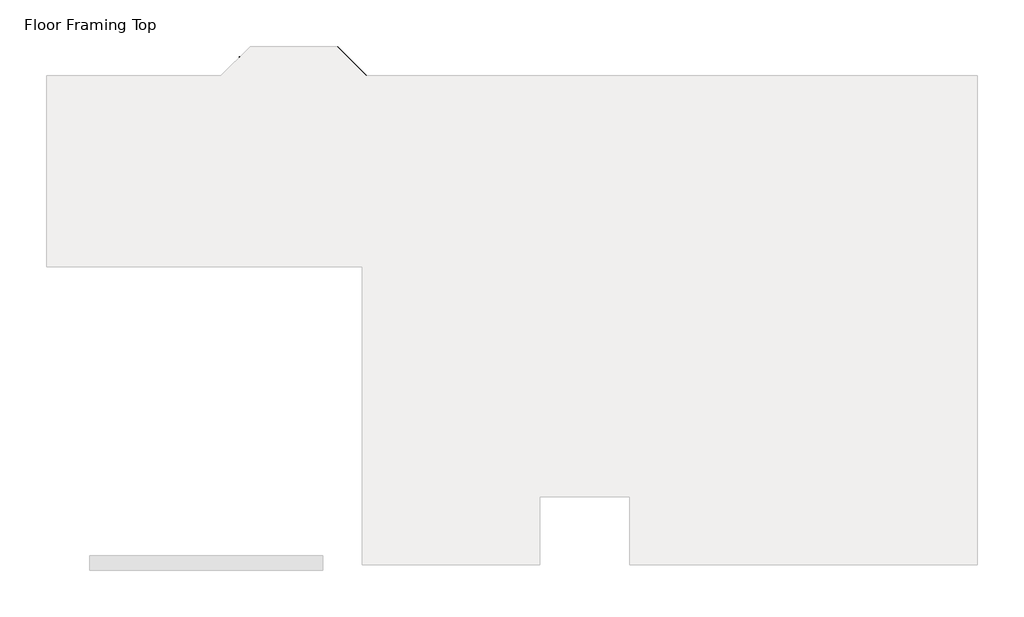
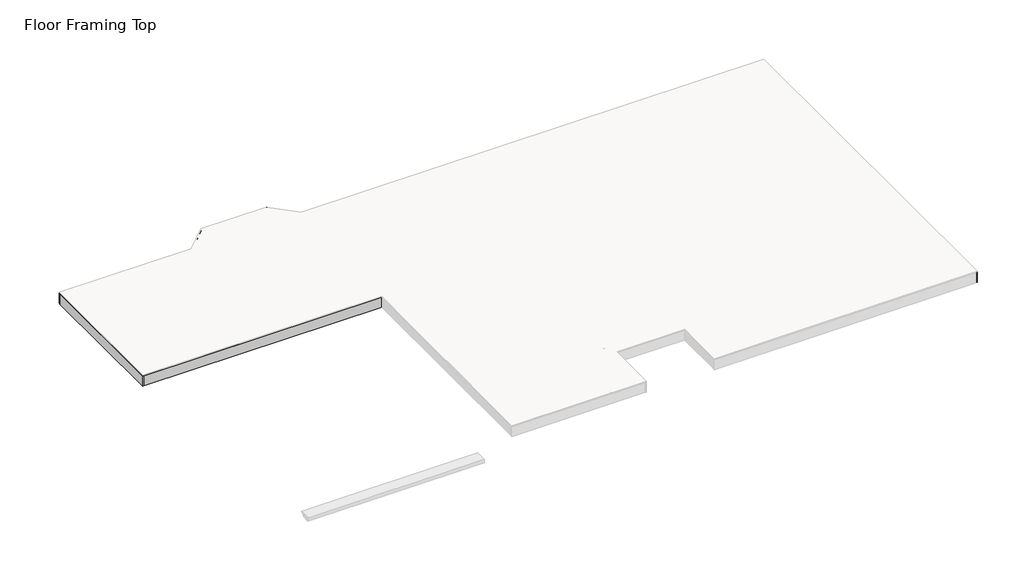
# One storey, part 4 of 4: 30 beams.
"""IFC4 building model written with IfcOpenShell, lengths in millimetres."""

import ifcopenshell
import ifcopenshell.guid

model = None  # the IFC model being written
_history = None  # IfcOwnerHistory: only IFC2X3 demands one
_inside = {}  # id of a spatial element -> (the spatial element, [elements in it])
_under = {}  # id of a project, library or spatial element -> (it, [spatial elements below it])
_declared = {}  # id of a project -> (the project, [libraries it declares])
_typed = {}  # id of a type object -> (the type object, [elements of that type])
_made_of = {}  # id of a material, layer set ... -> (it, [elements and type objects made of it])


def new_model(schema):
    """Start an empty IFC model of exactly this schema.

    Asked for "IFC4X3", IfcOpenShell would pick the latest addendum, in which some entities
    have other attributes; the version numbers below select the first issue.
    IFC2X3 requires an IfcOwnerHistory on every rooted entity: one is made here for all.
    """
    global model, _history
    if schema == "IFC4X3":
        model = ifcopenshell.file(schema_version=(4, 3, 0, 0))
    else:
        model = ifcopenshell.file(schema=schema)
    _inside.clear()
    _under.clear()
    _declared.clear()
    _typed.clear()
    _made_of.clear()
    _history = None
    if model.schema == "IFC2X3":
        org = make("IfcOrganization", Name="unknown")
        user = make(
            "IfcPersonAndOrganization",
            ThePerson=make("IfcPerson", FamilyName="unknown"),
            TheOrganization=org,
        )
        app = make(
            "IfcApplication",
            ApplicationDeveloper=org,
            Version="unknown",
            ApplicationFullName="unknown",
            ApplicationIdentifier="unknown",
        )
        _history = make(
            "IfcOwnerHistory",
            OwningUser=user,
            OwningApplication=app,
            ChangeAction="ADDED",
            CreationDate=0,
        )
    return model


def make(cls, **values):
    """One entity of the class cls with the attributes given. An attribute that is None is left unset."""
    return model.create_entity(
        cls, **{name: value for name, value in values.items() if value is not None}
    )


def rooted(cls, **values):
    """An entity with a GlobalId (a new one), such as an element, a storey or a relation."""
    return make(cls, GlobalId=ifcopenshell.guid.new(), OwnerHistory=_history, **values)


def si_unit(unit_type, name, prefix=None):
    """IfcSIUnit, for example si_unit("LENGTHUNIT", "METRE", prefix="MILLI")."""
    return make("IfcSIUnit", UnitType=unit_type, Prefix=prefix, Name=name)


def assignment(units):
    """IfcUnitAssignment: the units of a project."""
    return None if units is None else make("IfcUnitAssignment", Units=units)


def point(xyz):
    """IfcCartesianPoint."""
    return None if xyz is None else make("IfcCartesianPoint", Coordinates=xyz)


def direction(xyz):
    """IfcDirection."""
    return None if xyz is None else make("IfcDirection", DirectionRatios=xyz)


def frame(location, z_axis=None, x_axis=None):
    """IfcAxis2Placement3D, a coordinate frame: its origin and axes. An axis left out is left unset."""
    return make(
        "IfcAxis2Placement3D",
        Location=point(location),
        Axis=direction(z_axis),
        RefDirection=direction(x_axis),
    )


def origin():
    """The frame at (0, 0, 0) with its axes left unset."""
    return frame((0.0, 0.0, 0.0))


def place(relative_to, where):
    """IfcLocalPlacement: puts the frame where relative to a parent placement (None: the world)."""
    return make(
        "IfcLocalPlacement", PlacementRelTo=relative_to, RelativePlacement=where
    )


def context(
    kind, dimensions, precision=None, world=None, true_north=None, identifier=None
):
    """IfcGeometricRepresentationContext, for example the 3D "Model" context."""
    return make(
        "IfcGeometricRepresentationContext",
        ContextIdentifier=identifier,
        ContextType=kind,
        CoordinateSpaceDimension=dimensions,
        Precision=precision,
        WorldCoordinateSystem=world,
        TrueNorth=true_north,
    )


def project(units=None, contexts=None):
    """IfcProject with its units and contexts."""
    return rooted(
        "IfcProject",
        Name="project",
        RepresentationContexts=contexts,
        UnitsInContext=assignment(units),
    )


def spatial(cls, under=None, at=None, **own):
    """A site, building, storey or space (cls), placed at a placement, below another one or the project."""
    s = rooted(cls, ObjectPlacement=at, **own)
    if under is not None:
        _under.setdefault(under.id(), (under, []))[1].append(s)
    return s


def polyline(points):
    """IfcPolyline through the points."""
    return make("IfcPolyline", Points=[point(p) for p in points])


def outline(outer, holes=None, kind="AREA"):
    """IfcArbitraryClosedProfileDef: a profile drawn as a closed curve; with holes, ...WithVoids."""
    if holes is None:
        return make("IfcArbitraryClosedProfileDef", ProfileType=kind, OuterCurve=outer)
    return make(
        "IfcArbitraryProfileDefWithVoids",
        ProfileType=kind,
        OuterCurve=outer,
        InnerCurves=holes,
    )


def extrude(swept, where, along, depth):
    """IfcExtrudedAreaSolid: the profile swept, set in the frame where, extruded along a direction by depth."""
    return make(
        "IfcExtrudedAreaSolid",
        SweptArea=swept,
        Position=where,
        ExtrudedDirection=direction(along),
        Depth=depth,
    )


def faces_of(points, faces, orient=None, outer=None):
    """IfcFace entities. A face is a list of loops; a loop is a list of indices into points, from 0.

    orient and outer hold one flag for each loop. By default every Orientation is true, the
    first loop of a face is its IfcFaceOuterBound and the others are IfcFaceBound.
    """
    made = []
    for i, loops in enumerate(faces):
        bounds = []
        for j, loop in enumerate(loops):
            is_outer = j == 0 if outer is None else outer[i][j]
            bounds.append(
                make(
                    "IfcFaceOuterBound" if is_outer else "IfcFaceBound",
                    Bound=make("IfcPolyLoop", Polygon=[points[k] for k in loop]),
                    Orientation=True if orient is None else orient[i][j],
                )
            )
        made.append(make("IfcFace", Bounds=bounds))
    return made


def faceted_brep(points, faces, orient=None, outer=None, voids=None):
    """IfcFacetedBrep: a solid bounded by flat faces; with voids (closed shells), ...WithVoids."""
    shared = [point(p) for p in points]
    hull = make("IfcClosedShell", CfsFaces=faces_of(shared, faces, orient, outer))
    if voids is None:
        return make("IfcFacetedBrep", Outer=hull)
    return make(
        "IfcFacetedBrepWithVoids",
        Outer=hull,
        Voids=[
            make(cls, CfsFaces=faces_of(shared, fs, o, b)) for cls, fs, o, b in voids
        ],
    )


def shape(context_of_items, identifier, shape_type, items):
    """IfcShapeRepresentation: the items that make up one representation, for example the "Body"."""
    return make(
        "IfcShapeRepresentation",
        ContextOfItems=context_of_items,
        RepresentationIdentifier=identifier,
        RepresentationType=shape_type,
        Items=items,
    )


def source(mapping_origin, context_of_items, identifier, shape_type, items):
    """IfcRepresentationMap: a shape defined once, which mapped items show again and again."""
    return make(
        "IfcRepresentationMap",
        MappingOrigin=mapping_origin,
        MappedRepresentation=shape(context_of_items, identifier, shape_type, items),
    )


def transform(
    local_origin,
    x_axis=None,
    y_axis=None,
    z_axis=None,
    scale=None,
    scale2=None,
    scale3=None,
    uniform=True,
):
    """IfcCartesianTransformationOperator3D, or its non-uniform kind. x_axis, y_axis, z_axis: its Axis1, 2, 3."""
    if uniform:
        return make(
            "IfcCartesianTransformationOperator3D",
            Axis1=direction(x_axis),
            Axis2=direction(y_axis),
            LocalOrigin=point(local_origin),
            Scale=scale,
            Axis3=direction(z_axis),
        )
    return make(
        "IfcCartesianTransformationOperator3DnonUniform",
        Axis1=direction(x_axis),
        Axis2=direction(y_axis),
        LocalOrigin=point(local_origin),
        Scale=scale,
        Axis3=direction(z_axis),
        Scale2=scale2,
        Scale3=scale3,
    )


def mapped(mapping_source, mapping_target):
    """IfcMappedItem: shows the shape of a source again, moved by a transform."""
    return make(
        "IfcMappedItem", MappingSource=mapping_source, MappingTarget=mapping_target
    )


def made_of(thing, what):
    """Note that an element or type object is made of a material, layer set ...; save() writes the relation."""
    if what is not None:
        _made_of.setdefault(what.id(), (what, []))[1].append(thing)
    return thing


def element(
    cls,
    number,
    at=None,
    inside=None,
    cuts=None,
    type_object=None,
    material=None,
    context=None,
    identifier="Body",
    shape_type=None,
    held_by="IfcProductDefinitionShape",
    body=None,
    shapes=None,
    **own,
):
    """One element of the class cls, such as IfcWall. Its Tag is "e" and its number.

    at: its placement. inside: the storey or other place that contains it. cuts: it is an
    opening in that element (IfcRelVoidsElement). A single representation is given by context,
    identifier, shape_type and body (its items); several are given by shapes. held_by: the class
    of the entity that holds the representations. save() writes the other relations.
    """
    e = rooted(cls, Tag="e%d" % number, ObjectPlacement=at, **own)
    if body is not None:
        shapes = [shape(context, identifier, shape_type, body)]
    if shapes is not None:
        e.Representation = make(held_by, Representations=shapes)
    if inside is not None:
        _inside.setdefault(inside.id(), (inside, []))[1].append(e)
    if cuts is not None:
        rooted(
            "IfcRelVoidsElement", RelatingBuildingElement=cuts, RelatedOpeningElement=e
        )
    if type_object is not None:
        _typed.setdefault(type_object.id(), (type_object, []))[1].append(e)
    return made_of(e, material)


def aggregate(whole, parts):
    """IfcRelAggregates: a whole, such as a stair, and the parts it consists of."""
    return rooted("IfcRelAggregates", RelatingObject=whole, RelatedObjects=parts)


def save(model, path):
    """Write the relations noted so far, then the file.

    IfcRelAggregates (storeys below a building ...), IfcRelContainedInSpatialStructure (elements
    in a storey), IfcRelDefinesByType, IfcRelAssociatesMaterial and IfcRelDeclares: one each for
    every whole, place, type object, material and project.
    """
    for whole, parts in _under.values():
        aggregate(whole, parts)
    for where, things in _inside.values():
        rooted(
            "IfcRelContainedInSpatialStructure",
            RelatedElements=things,
            RelatingStructure=where,
        )
    for kind, things in _typed.values():
        rooted("IfcRelDefinesByType", RelatedObjects=things, RelatingType=kind)
    for what, things in _made_of.values():
        rooted("IfcRelAssociatesMaterial", RelatedObjects=things, RelatingMaterial=what)
    for by, libraries in _declared.values():
        rooted("IfcRelDeclares", RelatingContext=by, RelatedDefinitions=libraries)
    model.write(path)


def lvl_laminated_veneer_lumber_rim_board_13dc89ba(model_context):
    return source(origin(), model_context, "Body", "SweptSolid", [
        extrude(outline(polyline([(1981.99375, 15.875), (1981.99375, -15.875), (-1985.16875, -15.875), (-1985.16875, 15.875), (1981.99375, 15.875)])), frame((0.0, 0.0, -150.8125), z_axis=(0.0, 0.0, 1.0), x_axis=(1.0, 0.0, 0.0)), (0.0, 0.0, 1.0), 301.625),
    ])


def lvl_laminated_veneer_lumber_rim_board_6caa49f5(model_context):
    return source(origin(), model_context, "Body", "SweptSolid", [
        extrude(outline(polyline([(3288.50625, 15.875), (3288.50625, -15.875), (-3288.50625, -15.875), (-3288.50625, 15.875), (3288.50625, 15.875)])), frame((0.0, 0.0, -150.8125), z_axis=(0.0, 0.0, 1.0), x_axis=(1.0, 0.0, 0.0)), (0.0, 0.0, 1.0), 301.625),
    ])


def lvl_laminated_veneer_lumber_rim_board_c76fbf88(model_context):
    return source(origin(), model_context, "Body", "SweptSolid", [
        extrude(outline(polyline([(5118.89375, 15.875), (5118.89375, -15.875), (-5118.89375, -15.875), (-5118.89375, 15.875), (5118.89375, 15.875)])), frame((0.0, 0.0, -150.8125), z_axis=(0.0, 0.0, 1.0), x_axis=(1.0, 0.0, 0.0)), (0.0, 0.0, 1.0), 301.625),
    ])


def plywood_web_joist_11_7_8_tji_150_914fbb7f(model_context):
    return source(origin(), model_context, "Body", "SweptSolid", [
        extrude(outline(polyline([(-19.05, 150.8125), (19.05, 150.8125), (19.05, 112.7125), (4.7625, 112.7125), (4.7625, 119.0625), (-4.7625, 119.0625), (-4.7625, 112.7125), (-19.05, 112.7125), (-19.05, 150.8125)])), frame((-2272.50625, 0.0, 0.0), z_axis=(1.0, 0.0, 0.0), x_axis=(0.0, 1.0, 0.0)), (0.0, 0.0, 1.0), 4545.0125),
        extrude(outline(polyline([(19.05, -112.7125), (19.05, -150.8125), (-19.05, -150.8125), (-19.05, -112.7125), (-4.7625, -112.7125), (-4.7625, -118.3285374), (4.7625, -118.3285374), (4.7625, -112.7125), (19.05, -112.7125)])), frame((-2272.50625, 0.0, 0.0), z_axis=(1.0, 0.0, 0.0), x_axis=(0.0, 1.0, 0.0)), (0.0, 0.0, 1.0), 4545.0125),
        extrude(outline(polyline([(2272.50625, 4.7625), (2272.50625, -4.7625), (-2272.50625, -4.7625), (-2272.50625, 4.7625), (2272.50625, 4.7625)])), frame((0.0, 0.0, -118.3285374), z_axis=(0.0, 0.0, 1.0), x_axis=(1.0, 0.0, 0.0)), (0.0, 0.0, 1.0), 237.3910374),
    ])


def plywood_web_joist_11_7_8_tji_150_4ba6f87f(model_context):
    return source(origin(), model_context, "Body", "SweptSolid", [
        extrude(outline(polyline([(-19.05, 150.8125), (19.05, 150.8125), (19.05, 112.7125), (4.7625, 112.7125), (4.7625, 119.0625), (-4.7625, 119.0625), (-4.7625, 112.7125), (-19.05, 112.7125), (-19.05, 150.8125)])), frame((-1967.70625, 0.0, 0.0), z_axis=(1.0, 0.0, 0.0), x_axis=(0.0, 1.0, 0.0)), (0.0, 0.0, 1.0), 3935.4125),
        extrude(outline(polyline([(19.05, -112.7125), (19.05, -150.8125), (-19.05, -150.8125), (-19.05, -112.7125), (-4.7625, -112.7125), (-4.7625, -118.3285374), (4.7625, -118.3285374), (4.7625, -112.7125), (19.05, -112.7125)])), frame((-1967.70625, 0.0, 0.0), z_axis=(1.0, 0.0, 0.0), x_axis=(0.0, 1.0, 0.0)), (0.0, 0.0, 1.0), 3935.4125),
        extrude(outline(polyline([(1967.70625, 4.7625), (1967.70625, -4.7625), (-1967.70625, -4.7625), (-1967.70625, 4.7625), (1967.70625, 4.7625)])), frame((0.0, 0.0, -118.3285374), z_axis=(0.0, 0.0, 1.0), x_axis=(1.0, 0.0, 0.0)), (0.0, 0.0, 1.0), 237.3910374),
    ])


model = new_model("IFC4")

# Units and contexts
model_context = context("Model", 3, world=origin())
ifc_project = project(units=[si_unit("LENGTHUNIT", "METRE", prefix="MILLI")], contexts=[model_context])

# Site, building, storey
site = spatial("IfcSite", under=ifc_project)
building = spatial("IfcBuilding", under=site)
storey = spatial("IfcBuildingStorey", under=building, Name="Floor Framing Top", Elevation=0.0)

# Beams
placement = place(None, origin())
element("IfcBeam", 1, ObjectType="LVL-Laminated Veneer Lumber : Rim Board", at=placement, inside=storey, context=model_context, shape_type="SweptSolid", body=[
    extrude(outline(polyline([(-2583.3027251, 4488.2334053), (-2570.1514445, 4456.4834053), (-6240.9027251, 4456.4834053), (-6240.9027251, 4488.2334053), (-2583.3027251, 4488.2334053)])), frame((0.0, 0.0, -301.625), z_axis=(0.0, 0.0, 1.0), x_axis=(1.0, 0.0, 0.0)), (0.0, 0.0, 1.0), 301.625),
])
element("IfcBeam", 2, ObjectType="LVL-Laminated Veneer Lumber : Rim Board", at=placement, inside=storey, context=model_context, shape_type="SweptSolid", body=[
    extrude(outline(polyline([(-1973.7027251, 5097.8334053), (-1960.5514445, 5066.0834053), (-2570.1514445, 4456.4834053), (-2583.3027251, 4488.2334053), (-1973.7027251, 5097.8334053)])), frame((0.0, 0.0, -301.625), z_axis=(0.0, 0.0, 1.0), x_axis=(1.0, 0.0, 0.0)), (0.0, 0.0, 1.0), 301.625),
])
element("IfcBeam", 3, ObjectType="LVL-Laminated Veneer Lumber : Rim Board", at=placement, inside=storey, context=model_context, shape_type="SweptSolid", body=[
    extrude(outline(polyline([(-144.9027251, 5097.8334053), (-158.0540057, 5066.0834053), (-1960.5514445, 5066.0834053), (-1973.7027251, 5097.8334053), (-144.9027251, 5097.8334053)])), frame((0.0, 0.0, -301.625), z_axis=(0.0, 0.0, 1.0), x_axis=(1.0, 0.0, 0.0)), (0.0, 0.0, 1.0), 301.625),
])
element("IfcBeam", 4, ObjectType="LVL-Laminated Veneer Lumber : Rim Board", at=placement, inside=storey, context=model_context, shape_type="SweptSolid", body=[
    extrude(outline(polyline([(451.5459943, 4456.4834053), (464.6972749, 4488.2334053), (13212.3222749, 4488.2334053), (13212.3222749, 4456.4834053), (451.5459943, 4456.4834053)])), frame((0.0, 0.0, -301.625), z_axis=(0.0, 0.0, 1.0), x_axis=(1.0, 0.0, 0.0)), (0.0, 0.0, 1.0), 301.625),
])
element("IfcBeam", 5, ObjectType="LVL-Laminated Veneer Lumber : Rim Board", at=placement, inside=storey, context=model_context, shape_type="SweptSolid", body=[
    extrude(outline(polyline([(-144.9027251, 5097.8334053), (464.6972749, 4488.2334053), (451.5459943, 4456.4834053), (-158.0540057, 5066.0834053), (-144.9027251, 5097.8334053)])), frame((0.0, 0.0, -301.625), z_axis=(0.0, 0.0, 1.0), x_axis=(1.0, 0.0, 0.0)), (0.0, 0.0, 1.0), 301.625),
])
lvl_laminated_veneer_lumber_rim_board_shape = lvl_laminated_veneer_lumber_rim_board_13dc89ba(model_context)
element("IfcBeam", 6, ObjectType="LVL-Laminated Veneer Lumber : Rim Board", at=placement, inside=storey, context=model_context, shape_type="MappedRepresentation", body=[
    mapped(lvl_laminated_veneer_lumber_rim_board_shape, transform((-6225.0277251, 2471.3146553, -150.8125), x_axis=(0.0, -1.0, 0.0), y_axis=(1.0, 0.0, 0.0), z_axis=(0.0, 0.0, 1.0))),
])
lvl_laminated_veneer_lumber_rim_board_2_shape = lvl_laminated_veneer_lumber_rim_board_6caa49f5(model_context)
element("IfcBeam", 7, ObjectType="LVL-Laminated Veneer Lumber : Rim Board", at=placement, inside=storey, context=model_context, shape_type="MappedRepresentation", body=[
    mapped(lvl_laminated_veneer_lumber_rim_board_2_shape, transform((-2920.6464751, 505.1959053, -150.8125), x_axis=(1.0, 0.0, 0.0), y_axis=(0.0, 1.0, 0.0), z_axis=(0.0, 0.0, 1.0))),
])
lvl_laminated_veneer_lumber_rim_board_3_shape = lvl_laminated_veneer_lumber_rim_board_c76fbf88(model_context)
element("IfcBeam", 8, ObjectType="LVL-Laminated Veneer Lumber : Rim Board", at=placement, inside=storey, context=model_context, shape_type="MappedRepresentation", body=[
    mapped(lvl_laminated_veneer_lumber_rim_board_3_shape, transform((13228.1972749, -630.6603447, -150.8125), x_axis=(0.0, 1.0, 0.0), y_axis=(-1.0, 0.0, 0.0), z_axis=(0.0, 0.0, 1.0))),
])
element("IfcBeam", 9, ObjectType="Plywood Web Joist : 11 7/8 TJI 150", at=placement, inside=storey, context=model_context, shape_type="SweptSolid", body=[
    extrude(outline(polyline([(12040.7472749, -5717.8040947), (12031.2222749, -5717.8040947), (12031.2222749, 4456.4834053), (12040.7472749, 4456.4834053), (12040.7472749, -5717.8040947)])), frame((0.0, 0.0, -269.1410374), z_axis=(0.0, 0.0, 1.0), x_axis=(1.0, 0.0, 0.0)), (0.0, 0.0, 1.0), 237.3910374),
    extrude(outline(polyline([(12031.2222749, -663.2040947), (12031.2222749, 4456.4834053), (12040.7472749, 4456.4834053), (12040.7472749, -663.2040947), (12031.2222749, -663.2040947)])), frame((0.0, 0.0, -269.1410374), z_axis=(0.0, 0.0, 1.0), x_axis=(1.0, 0.0, 0.0)), (0.0, 0.0, 1.0), 237.3910374),
    extrude(outline(polyline([(0.0, 12016.9347749), (-38.1, 12016.9347749), (-38.1, 12031.2222749), (-31.75, 12031.2222749), (-31.75, 12040.7472749), (-38.1, 12040.7472749), (-38.1, 12055.0347749), (0.0, 12055.0347749), (0.0, 12016.9347749)])), frame((0.0, -5717.8040947, 0.0), z_axis=(0.0, 1.0, 0.0), x_axis=(0.0, 0.0, 1.0)), (0.0, 0.0, 1.0), 10174.2875),
    extrude(outline(polyline([(-263.525, 12055.0347749), (-263.525, 12040.7472749), (-269.1410374, 12040.7472749), (-269.1410374, 12031.2222749), (-263.525, 12031.2222749), (-263.525, 12016.9347749), (-301.625, 12016.9347749), (-301.625, 12055.0347749), (-263.525, 12055.0347749)])), frame((0.0, -5717.8040947, 0.0), z_axis=(0.0, 1.0, 0.0), x_axis=(0.0, 0.0, 1.0)), (0.0, 0.0, 1.0), 10174.2875),
    extrude(outline(polyline([(0.0, 12016.9347749), (-38.1, 12016.9347749), (-38.1, 12031.2222749), (-31.75, 12031.2222749), (-31.75, 12040.7472749), (-38.1, 12040.7472749), (-38.1, 12055.0347749), (0.0, 12055.0347749), (0.0, 12016.9347749)])), frame((0.0, -663.2040947, 0.0), z_axis=(0.0, 1.0, 0.0), x_axis=(0.0, 0.0, 1.0)), (0.0, 0.0, 1.0), 5119.6875),
    extrude(outline(polyline([(-263.525, 12055.0347749), (-263.525, 12040.7472749), (-269.1410374, 12040.7472749), (-269.1410374, 12031.2222749), (-263.525, 12031.2222749), (-263.525, 12016.9347749), (-301.625, 12016.9347749), (-301.625, 12055.0347749), (-263.525, 12055.0347749)])), frame((0.0, -663.2040947, 0.0), z_axis=(0.0, 1.0, 0.0), x_axis=(0.0, 0.0, 1.0)), (0.0, 0.0, 1.0), 5119.6875),
])
element("IfcBeam", 10, ObjectType="Plywood Web Joist : 11 7/8 TJI 150", at=placement, inside=storey, context=model_context, shape_type="SweptSolid", body=[
    extrude(outline(polyline([(5944.7472749, -4295.4040947), (5935.2222749, -4295.4040947), (5935.2222749, 4456.4834053), (5944.7472749, 4456.4834053), (5944.7472749, -4295.4040947)])), frame((0.0, 0.0, -269.1410374), z_axis=(0.0, 0.0, 1.0), x_axis=(1.0, 0.0, 0.0)), (0.0, 0.0, 1.0), 237.3910374),
    extrude(outline(polyline([(5935.2222749, -663.2040947), (5935.2222749, 4456.4834053), (5944.7472749, 4456.4834053), (5944.7472749, -663.2040947), (5935.2222749, -663.2040947)])), frame((0.0, 0.0, -269.1410374), z_axis=(0.0, 0.0, 1.0), x_axis=(1.0, 0.0, 0.0)), (0.0, 0.0, 1.0), 237.3910374),
    extrude(outline(polyline([(0.0, 5920.9347749), (-38.1, 5920.9347749), (-38.1, 5935.2222749), (-31.75, 5935.2222749), (-31.75, 5944.7472749), (-38.1, 5944.7472749), (-38.1, 5959.0347749), (0.0, 5959.0347749), (0.0, 5920.9347749)])), frame((0.0, -4295.4040947, 0.0), z_axis=(0.0, 1.0, 0.0), x_axis=(0.0, 0.0, 1.0)), (0.0, 0.0, 1.0), 8751.8875),
    extrude(outline(polyline([(-263.525, 5959.0347749), (-263.525, 5944.7472749), (-269.1410374, 5944.7472749), (-269.1410374, 5935.2222749), (-263.525, 5935.2222749), (-263.525, 5920.9347749), (-301.625, 5920.9347749), (-301.625, 5959.0347749), (-263.525, 5959.0347749)])), frame((0.0, -4295.4040947, 0.0), z_axis=(0.0, 1.0, 0.0), x_axis=(0.0, 0.0, 1.0)), (0.0, 0.0, 1.0), 8751.8875),
    extrude(outline(polyline([(0.0, 5920.9347749), (-38.1, 5920.9347749), (-38.1, 5935.2222749), (-31.75, 5935.2222749), (-31.75, 5944.7472749), (-38.1, 5944.7472749), (-38.1, 5959.0347749), (0.0, 5959.0347749), (0.0, 5920.9347749)])), frame((0.0, -663.2040947, 0.0), z_axis=(0.0, 1.0, 0.0), x_axis=(0.0, 0.0, 1.0)), (0.0, 0.0, 1.0), 5119.6875),
    extrude(outline(polyline([(-263.525, 5959.0347749), (-263.525, 5944.7472749), (-269.1410374, 5944.7472749), (-269.1410374, 5935.2222749), (-263.525, 5935.2222749), (-263.525, 5920.9347749), (-301.625, 5920.9347749), (-301.625, 5959.0347749), (-263.525, 5959.0347749)])), frame((0.0, -663.2040947, 0.0), z_axis=(0.0, 1.0, 0.0), x_axis=(0.0, 0.0, 1.0)), (0.0, 0.0, 1.0), 5119.6875),
])
element("IfcBeam", 11, ObjectType="Plywood Web Joist : 11 7/8 TJI 150", at=placement, inside=storey, context=model_context, shape_type="SweptSolid", body=[
    extrude(outline(polyline([(5538.3472749, -4295.4040947), (5528.8222749, -4295.4040947), (5528.8222749, 4456.4834053), (5538.3472749, 4456.4834053), (5538.3472749, -4295.4040947)])), frame((0.0, 0.0, -269.1410374), z_axis=(0.0, 0.0, 1.0), x_axis=(1.0, 0.0, 0.0)), (0.0, 0.0, 1.0), 237.3910374),
    extrude(outline(polyline([(5528.8222749, -663.2040947), (5528.8222749, 4456.4834053), (5538.3472749, 4456.4834053), (5538.3472749, -663.2040947), (5528.8222749, -663.2040947)])), frame((0.0, 0.0, -269.1410374), z_axis=(0.0, 0.0, 1.0), x_axis=(1.0, 0.0, 0.0)), (0.0, 0.0, 1.0), 237.3910374),
    extrude(outline(polyline([(0.0, 5514.5347749), (-38.1, 5514.5347749), (-38.1, 5528.8222749), (-31.75, 5528.8222749), (-31.75, 5538.3472749), (-38.1, 5538.3472749), (-38.1, 5552.6347749), (0.0, 5552.6347749), (0.0, 5514.5347749)])), frame((0.0, -4295.4040947, 0.0), z_axis=(0.0, 1.0, 0.0), x_axis=(0.0, 0.0, 1.0)), (0.0, 0.0, 1.0), 8751.8875),
    extrude(outline(polyline([(-263.525, 5552.6347749), (-263.525, 5538.3472749), (-269.1410374, 5538.3472749), (-269.1410374, 5528.8222749), (-263.525, 5528.8222749), (-263.525, 5514.5347749), (-301.625, 5514.5347749), (-301.625, 5552.6347749), (-263.525, 5552.6347749)])), frame((0.0, -4295.4040947, 0.0), z_axis=(0.0, 1.0, 0.0), x_axis=(0.0, 0.0, 1.0)), (0.0, 0.0, 1.0), 8751.8875),
    extrude(outline(polyline([(0.0, 5514.5347749), (-38.1, 5514.5347749), (-38.1, 5528.8222749), (-31.75, 5528.8222749), (-31.75, 5538.3472749), (-38.1, 5538.3472749), (-38.1, 5552.6347749), (0.0, 5552.6347749), (0.0, 5514.5347749)])), frame((0.0, -663.2040947, 0.0), z_axis=(0.0, 1.0, 0.0), x_axis=(0.0, 0.0, 1.0)), (0.0, 0.0, 1.0), 5119.6875),
    extrude(outline(polyline([(-263.525, 5552.6347749), (-263.525, 5538.3472749), (-269.1410374, 5538.3472749), (-269.1410374, 5528.8222749), (-263.525, 5528.8222749), (-263.525, 5514.5347749), (-301.625, 5514.5347749), (-301.625, 5552.6347749), (-263.525, 5552.6347749)])), frame((0.0, -663.2040947, 0.0), z_axis=(0.0, 1.0, 0.0), x_axis=(0.0, 0.0, 1.0)), (0.0, 0.0, 1.0), 5119.6875),
])
element("IfcBeam", 12, ObjectType="Plywood Web Joist : 11 7/8 TJI 150", at=placement, inside=storey, context=model_context, shape_type="SweptSolid", body=[
    extrude(outline(polyline([(5131.9472749, -4295.4040947), (5122.4222749, -4295.4040947), (5122.4222749, 4456.4834053), (5131.9472749, 4456.4834053), (5131.9472749, -4295.4040947)])), frame((0.0, 0.0, -269.1410374), z_axis=(0.0, 0.0, 1.0), x_axis=(1.0, 0.0, 0.0)), (0.0, 0.0, 1.0), 237.3910374),
    extrude(outline(polyline([(5122.4222749, -663.2040947), (5122.4222749, 4456.4834053), (5131.9472749, 4456.4834053), (5131.9472749, -663.2040947), (5122.4222749, -663.2040947)])), frame((0.0, 0.0, -269.1410374), z_axis=(0.0, 0.0, 1.0), x_axis=(1.0, 0.0, 0.0)), (0.0, 0.0, 1.0), 237.3910374),
    extrude(outline(polyline([(0.0, 5108.1347749), (-38.1, 5108.1347749), (-38.1, 5122.4222749), (-31.75, 5122.4222749), (-31.75, 5131.9472749), (-38.1, 5131.9472749), (-38.1, 5146.2347749), (0.0, 5146.2347749), (0.0, 5108.1347749)])), frame((0.0, -4295.4040947, 0.0), z_axis=(0.0, 1.0, 0.0), x_axis=(0.0, 0.0, 1.0)), (0.0, 0.0, 1.0), 8751.8875),
    extrude(outline(polyline([(-263.525, 5146.2347749), (-263.525, 5131.9472749), (-269.1410374, 5131.9472749), (-269.1410374, 5122.4222749), (-263.525, 5122.4222749), (-263.525, 5108.1347749), (-301.625, 5108.1347749), (-301.625, 5146.2347749), (-263.525, 5146.2347749)])), frame((0.0, -4295.4040947, 0.0), z_axis=(0.0, 1.0, 0.0), x_axis=(0.0, 0.0, 1.0)), (0.0, 0.0, 1.0), 8751.8875),
    extrude(outline(polyline([(0.0, 5108.1347749), (-38.1, 5108.1347749), (-38.1, 5122.4222749), (-31.75, 5122.4222749), (-31.75, 5131.9472749), (-38.1, 5131.9472749), (-38.1, 5146.2347749), (0.0, 5146.2347749), (0.0, 5108.1347749)])), frame((0.0, -663.2040947, 0.0), z_axis=(0.0, 1.0, 0.0), x_axis=(0.0, 0.0, 1.0)), (0.0, 0.0, 1.0), 5119.6875),
    extrude(outline(polyline([(-263.525, 5146.2347749), (-263.525, 5131.9472749), (-269.1410374, 5131.9472749), (-269.1410374, 5122.4222749), (-263.525, 5122.4222749), (-263.525, 5108.1347749), (-301.625, 5108.1347749), (-301.625, 5146.2347749), (-263.525, 5146.2347749)])), frame((0.0, -663.2040947, 0.0), z_axis=(0.0, 1.0, 0.0), x_axis=(0.0, 0.0, 1.0)), (0.0, 0.0, 1.0), 5119.6875),
])
element("IfcBeam", 13, ObjectType="Plywood Web Joist : 11 7/8 TJI 150", at=placement, inside=storey, context=model_context, shape_type="SweptSolid", body=[
    extrude(outline(polyline([(4725.5472749, -4295.4040947), (4716.0222749, -4295.4040947), (4716.0222749, 4456.4834053), (4725.5472749, 4456.4834053), (4725.5472749, -4295.4040947)])), frame((0.0, 0.0, -269.1410374), z_axis=(0.0, 0.0, 1.0), x_axis=(1.0, 0.0, 0.0)), (0.0, 0.0, 1.0), 237.3910374),
    extrude(outline(polyline([(4716.0222749, -663.2040947), (4716.0222749, 4456.4834053), (4725.5472749, 4456.4834053), (4725.5472749, -663.2040947), (4716.0222749, -663.2040947)])), frame((0.0, 0.0, -269.1410374), z_axis=(0.0, 0.0, 1.0), x_axis=(1.0, 0.0, 0.0)), (0.0, 0.0, 1.0), 237.3910374),
    extrude(outline(polyline([(0.0, 4701.7347749), (-38.1, 4701.7347749), (-38.1, 4716.0222749), (-31.75, 4716.0222749), (-31.75, 4725.5472749), (-38.1, 4725.5472749), (-38.1, 4739.8347749), (0.0, 4739.8347749), (0.0, 4701.7347749)])), frame((0.0, -4295.4040947, 0.0), z_axis=(0.0, 1.0, 0.0), x_axis=(0.0, 0.0, 1.0)), (0.0, 0.0, 1.0), 8751.8875),
    extrude(outline(polyline([(-263.525, 4739.8347749), (-263.525, 4725.5472749), (-269.1410374, 4725.5472749), (-269.1410374, 4716.0222749), (-263.525, 4716.0222749), (-263.525, 4701.7347749), (-301.625, 4701.7347749), (-301.625, 4739.8347749), (-263.525, 4739.8347749)])), frame((0.0, -4295.4040947, 0.0), z_axis=(0.0, 1.0, 0.0), x_axis=(0.0, 0.0, 1.0)), (0.0, 0.0, 1.0), 8751.8875),
    extrude(outline(polyline([(0.0, 4701.7347749), (-38.1, 4701.7347749), (-38.1, 4716.0222749), (-31.75, 4716.0222749), (-31.75, 4725.5472749), (-38.1, 4725.5472749), (-38.1, 4739.8347749), (0.0, 4739.8347749), (0.0, 4701.7347749)])), frame((0.0, -663.2040947, 0.0), z_axis=(0.0, 1.0, 0.0), x_axis=(0.0, 0.0, 1.0)), (0.0, 0.0, 1.0), 5119.6875),
    extrude(outline(polyline([(-263.525, 4739.8347749), (-263.525, 4725.5472749), (-269.1410374, 4725.5472749), (-269.1410374, 4716.0222749), (-263.525, 4716.0222749), (-263.525, 4701.7347749), (-301.625, 4701.7347749), (-301.625, 4739.8347749), (-263.525, 4739.8347749)])), frame((0.0, -663.2040947, 0.0), z_axis=(0.0, 1.0, 0.0), x_axis=(0.0, 0.0, 1.0)), (0.0, 0.0, 1.0), 5119.6875),
])
element("IfcBeam", 14, ObjectType="Plywood Web Joist : 11 7/8 TJI 150", at=placement, inside=storey, context=model_context, shape_type="SweptSolid", body=[
    extrude(outline(polyline([(4319.1472749, -4295.4040947), (4309.6222749, -4295.4040947), (4309.6222749, 4456.4834053), (4319.1472749, 4456.4834053), (4319.1472749, -4295.4040947)])), frame((0.0, 0.0, -269.1410374), z_axis=(0.0, 0.0, 1.0), x_axis=(1.0, 0.0, 0.0)), (0.0, 0.0, 1.0), 237.3910374),
    extrude(outline(polyline([(4309.6222749, -663.2040947), (4309.6222749, 4456.4834053), (4319.1472749, 4456.4834053), (4319.1472749, -663.2040947), (4309.6222749, -663.2040947)])), frame((0.0, 0.0, -269.1410374), z_axis=(0.0, 0.0, 1.0), x_axis=(1.0, 0.0, 0.0)), (0.0, 0.0, 1.0), 237.3910374),
    extrude(outline(polyline([(0.0, 4295.3347749), (-38.1, 4295.3347749), (-38.1, 4309.6222749), (-31.75, 4309.6222749), (-31.75, 4319.1472749), (-38.1, 4319.1472749), (-38.1, 4333.4347749), (0.0, 4333.4347749), (0.0, 4295.3347749)])), frame((0.0, -4295.4040947, 0.0), z_axis=(0.0, 1.0, 0.0), x_axis=(0.0, 0.0, 1.0)), (0.0, 0.0, 1.0), 8751.8875),
    extrude(outline(polyline([(-263.525, 4333.4347749), (-263.525, 4319.1472749), (-269.1410374, 4319.1472749), (-269.1410374, 4309.6222749), (-263.525, 4309.6222749), (-263.525, 4295.3347749), (-301.625, 4295.3347749), (-301.625, 4333.4347749), (-263.525, 4333.4347749)])), frame((0.0, -4295.4040947, 0.0), z_axis=(0.0, 1.0, 0.0), x_axis=(0.0, 0.0, 1.0)), (0.0, 0.0, 1.0), 8751.8875),
    extrude(outline(polyline([(0.0, 4295.3347749), (-38.1, 4295.3347749), (-38.1, 4309.6222749), (-31.75, 4309.6222749), (-31.75, 4319.1472749), (-38.1, 4319.1472749), (-38.1, 4333.4347749), (0.0, 4333.4347749), (0.0, 4295.3347749)])), frame((0.0, -663.2040947, 0.0), z_axis=(0.0, 1.0, 0.0), x_axis=(0.0, 0.0, 1.0)), (0.0, 0.0, 1.0), 5119.6875),
    extrude(outline(polyline([(-263.525, 4333.4347749), (-263.525, 4319.1472749), (-269.1410374, 4319.1472749), (-269.1410374, 4309.6222749), (-263.525, 4309.6222749), (-263.525, 4295.3347749), (-301.625, 4295.3347749), (-301.625, 4333.4347749), (-263.525, 4333.4347749)])), frame((0.0, -663.2040947, 0.0), z_axis=(0.0, 1.0, 0.0), x_axis=(0.0, 0.0, 1.0)), (0.0, 0.0, 1.0), 5119.6875),
])
element("IfcBeam", 15, ObjectType="Plywood Web Joist : 11 7/8 TJI 150", at=placement, inside=storey, context=model_context, shape_type="SolidModel", body=[
    extrude(outline(polyline([(255.1472749, 521.0709053), (245.6222749, 521.0709053), (245.6222749, 4676.3276256), (255.1472749, 4676.3276256), (255.1472749, 521.0709053)])), frame((0.0, 0.0, -269.1410374), z_axis=(0.0, 0.0, 1.0), x_axis=(1.0, 0.0, 0.0)), (0.0, 0.0, 1.0), 237.3910374),
    extrude(outline(polyline([(255.1472749, 521.0709053), (245.6222749, 521.0709053), (245.6222749, 4662.4071247), (255.1472749, 4652.8821247), (255.1472749, 521.0709053)])), frame((0.0, 0.0, -269.1410374), z_axis=(0.0, 0.0, 1.0), x_axis=(1.0, 0.0, 0.0)), (0.0, 0.0, 1.0), 237.3910374),
    faceted_brep([(231.3347749, 521.0709053, 0.0), (231.3347749, 521.0709053, -38.1), (245.6222749, 521.0709053, -38.1), (245.6222749, 521.0709053, -31.75), (255.1472749, 521.0709053, -31.75), (255.1472749, 521.0709053, -38.1), (269.4347749, 521.0709053, -38.1), (269.4347749, 521.0709053, 0.0), (231.3347749, 4676.3276256, 0.0), (269.4347749, 4676.3276256, 0.0), (269.4347749, 4676.3276256, -38.1), (255.1472749, 4676.3276256, -38.1), (255.1472749, 4676.3276256, -31.75), (245.6222749, 4676.3276256, -31.75), (245.6222749, 4676.3276256, -38.1), (231.3347749, 4676.3276256, -38.1)], [[[0, 1, 2, 3, 4, 5, 6, 7]], [[8, 9, 10, 11, 12, 13, 14, 15]], [[1, 0, 8, 15]], [[2, 1, 15, 14]], [[3, 2, 14, 13]], [[4, 3, 13, 12]], [[5, 4, 12, 11]], [[6, 5, 11, 10]], [[7, 6, 10, 9]], [[0, 7, 9, 8]]]),
    faceted_brep([(269.4347749, 521.0709053, -263.525), (255.1472749, 521.0709053, -263.525), (255.1472749, 521.0709053, -269.1410374), (245.6222749, 521.0709053, -269.1410374), (245.6222749, 521.0709053, -263.525), (231.3347749, 521.0709053, -263.525), (231.3347749, 521.0709053, -301.625), (269.4347749, 521.0709053, -301.625), (269.4347749, 4676.3276256, -263.525), (269.4347749, 4676.3276256, -301.625), (231.3347749, 4676.3276256, -301.625), (231.3347749, 4676.3276256, -263.525), (245.6222749, 4676.3276256, -263.525), (245.6222749, 4676.3276256, -269.1410374), (255.1472749, 4676.3276256, -269.1410374), (255.1472749, 4676.3276256, -263.525)], [[[0, 1, 2, 3, 4, 5, 6, 7]], [[8, 9, 10, 11, 12, 13, 14, 15]], [[1, 0, 8, 15]], [[2, 1, 15, 14]], [[3, 2, 14, 13]], [[4, 3, 13, 12]], [[5, 4, 12, 11]], [[6, 5, 11, 10]], [[7, 6, 10, 9]], [[0, 7, 9, 8]]]),
    faceted_brep([(231.7017739, 4676.3276256, -301.625), (231.7017739, 4676.3276256, -263.525), (245.6222749, 4662.4071247, -263.525), (245.6222749, 4662.4071247, -269.1410374), (255.1472749, 4652.8821247, -269.1410374), (255.1472749, 4652.8821247, -263.525), (269.4347749, 4638.5946247, -263.525), (269.4347749, 4638.5946247, -301.625), (269.4347749, 521.0709053, -263.525), (255.1472749, 521.0709053, -263.525), (255.1472749, 521.0709053, -269.1410374), (245.6222749, 521.0709053, -269.1410374), (245.6222749, 521.0709053, -263.525), (231.3347749, 521.0709053, -263.525), (231.3347749, 521.0709053, -301.625), (269.4347749, 521.0709053, -301.625), (231.3347749, 4676.3276256, -263.525), (231.3347749, 4676.3276256, -301.625)], [[[0, 1, 2, 3, 4, 5, 6, 7]], [[8, 9, 10, 11, 12, 13, 14, 15]], [[9, 8, 6, 5]], [[10, 9, 5, 4]], [[11, 10, 4, 3]], [[12, 11, 3, 2]], [[13, 12, 2, 1, 16]], [[14, 13, 16, 17]], [[15, 14, 17, 0, 7]], [[8, 15, 7, 6]], [[0, 17, 16, 1]]]),
    faceted_brep([(231.7017739, 4676.3276256, -38.1), (231.7017739, 4676.3276256, 0.0), (269.4347749, 4638.5946247, 0.0), (269.4347749, 4638.5946247, -38.1), (255.1472749, 4652.8821247, -38.1), (255.1472749, 4652.8821247, -31.75), (245.6222749, 4662.4071247, -31.75), (245.6222749, 4662.4071247, -38.1), (231.3347749, 521.0709053, 0.0), (231.3347749, 521.0709053, -38.1), (245.6222749, 521.0709053, -38.1), (245.6222749, 521.0709053, -31.75), (255.1472749, 521.0709053, -31.75), (255.1472749, 521.0709053, -38.1), (269.4347749, 521.0709053, -38.1), (269.4347749, 521.0709053, 0.0), (231.3347749, 4676.3276256, 0.0), (231.3347749, 4676.3276256, -38.1)], [[[0, 1, 2, 3, 4, 5, 6, 7]], [[8, 9, 10, 11, 12, 13, 14, 15]], [[9, 8, 16, 17]], [[10, 9, 17, 0, 7]], [[11, 10, 7, 6]], [[12, 11, 6, 5]], [[13, 12, 5, 4]], [[14, 13, 4, 3]], [[15, 14, 3, 2]], [[8, 15, 2, 1, 16]], [[16, 1, 0, 17]]]),
])
element("IfcBeam", 16, ObjectType="Plywood Web Joist : 11 7/8 TJI 150", at=placement, inside=storey, context=model_context, shape_type="SolidModel", body=[
    extrude(outline(polyline([(-151.2527251, 521.0709053), (-160.7777251, 521.0709053), (-160.7777251, 5066.0834053), (-151.2527251, 5066.0834053), (-151.2527251, 521.0709053)])), frame((0.0, 0.0, -269.1410374), z_axis=(0.0, 0.0, 1.0), x_axis=(1.0, 0.0, 0.0)), (0.0, 0.0, 1.0), 237.3910374),
    extrude(outline(polyline([(-151.2527251, 521.0709053), (-160.7777251, 521.0709053), (-160.7777251, 5066.0834053), (-158.0540057, 5066.0834053), (-151.2527251, 5059.2821247), (-151.2527251, 521.0709053)])), frame((0.0, 0.0, -269.1410374), z_axis=(0.0, 0.0, 1.0), x_axis=(1.0, 0.0, 0.0)), (0.0, 0.0, 1.0), 237.3910374),
    faceted_brep([(-175.0652251, 521.0709053, 0.0), (-175.0652251, 521.0709053, -38.1), (-160.7777251, 521.0709053, -38.1), (-160.7777251, 521.0709053, -31.75), (-151.2527251, 521.0709053, -31.75), (-151.2527251, 521.0709053, -38.1), (-136.9652251, 521.0709053, -38.1), (-136.9652251, 521.0709053, 0.0), (-175.0652251, 5066.0834053, 0.0), (-136.9652251, 5066.0834053, 0.0), (-136.9652251, 5066.0834053, -38.1), (-151.2527251, 5066.0834053, -38.1), (-151.2527251, 5066.0834053, -31.75), (-160.7777251, 5066.0834053, -31.75), (-160.7777251, 5066.0834053, -38.1), (-175.0652251, 5066.0834053, -38.1)], [[[0, 1, 2, 3, 4, 5, 6, 7]], [[8, 9, 10, 11, 12, 13, 14, 15]], [[1, 0, 8, 15]], [[2, 1, 15, 14]], [[3, 2, 14, 13]], [[4, 3, 13, 12]], [[5, 4, 12, 11]], [[6, 5, 11, 10]], [[7, 6, 10, 9]], [[0, 7, 9, 8]]]),
    faceted_brep([(-136.9652251, 521.0709053, -263.525), (-151.2527251, 521.0709053, -263.525), (-151.2527251, 521.0709053, -269.1410374), (-160.7777251, 521.0709053, -269.1410374), (-160.7777251, 521.0709053, -263.525), (-175.0652251, 521.0709053, -263.525), (-175.0652251, 521.0709053, -301.625), (-136.9652251, 521.0709053, -301.625), (-136.9652251, 5066.0834053, -263.525), (-136.9652251, 5066.0834053, -301.625), (-175.0652251, 5066.0834053, -301.625), (-175.0652251, 5066.0834053, -263.525), (-160.7777251, 5066.0834053, -263.525), (-160.7777251, 5066.0834053, -269.1410374), (-151.2527251, 5066.0834053, -269.1410374), (-151.2527251, 5066.0834053, -263.525)], [[[0, 1, 2, 3, 4, 5, 6, 7]], [[8, 9, 10, 11, 12, 13, 14, 15]], [[1, 0, 8, 15]], [[2, 1, 15, 14]], [[3, 2, 14, 13]], [[4, 3, 13, 12]], [[5, 4, 12, 11]], [[6, 5, 11, 10]], [[7, 6, 10, 9]], [[0, 7, 9, 8]]]),
    faceted_brep([(-158.0540057, 5066.0834053, -301.625), (-158.0540057, 5066.0834053, -269.1410374), (-151.2527251, 5059.2821247, -269.1410374), (-151.2527251, 5059.2821247, -263.525), (-136.9652251, 5044.9946247, -263.525), (-136.9652251, 5044.9946247, -301.625), (-136.9652251, 521.0709053, -263.525), (-151.2527251, 521.0709053, -263.525), (-151.2527251, 521.0709053, -269.1410374), (-160.7777251, 521.0709053, -269.1410374), (-160.7777251, 521.0709053, -263.525), (-175.0652251, 521.0709053, -263.525), (-175.0652251, 521.0709053, -301.625), (-136.9652251, 521.0709053, -301.625), (-160.7777251, 5066.0834053, -269.1410374), (-160.7777251, 5066.0834053, -263.525), (-175.0652251, 5066.0834053, -263.525), (-175.0652251, 5066.0834053, -301.625)], [[[0, 1, 2, 3, 4, 5]], [[6, 7, 8, 9, 10, 11, 12, 13]], [[7, 6, 4, 3]], [[8, 7, 3, 2]], [[9, 8, 2, 1, 14]], [[10, 9, 14, 15]], [[11, 10, 15, 16]], [[12, 11, 16, 17]], [[13, 12, 17, 0, 5]], [[6, 13, 5, 4]], [[0, 17, 16, 15, 14, 1]]]),
    faceted_brep([(-158.0540057, 5066.0834053, -31.75), (-158.0540057, 5066.0834053, 0.0), (-136.9652251, 5044.9946247, 0.0), (-136.9652251, 5044.9946247, -38.1), (-151.2527251, 5059.2821247, -38.1), (-151.2527251, 5059.2821247, -31.75), (-175.0652251, 521.0709053, 0.0), (-175.0652251, 521.0709053, -38.1), (-160.7777251, 521.0709053, -38.1), (-160.7777251, 521.0709053, -31.75), (-151.2527251, 521.0709053, -31.75), (-151.2527251, 521.0709053, -38.1), (-136.9652251, 521.0709053, -38.1), (-136.9652251, 521.0709053, 0.0), (-175.0652251, 5066.0834053, 0.0), (-175.0652251, 5066.0834053, -38.1), (-160.7777251, 5066.0834053, -38.1), (-160.7777251, 5066.0834053, -31.75)], [[[0, 1, 2, 3, 4, 5]], [[6, 7, 8, 9, 10, 11, 12, 13]], [[7, 6, 14, 15]], [[8, 7, 15, 16]], [[9, 8, 16, 17]], [[10, 9, 17, 0, 5]], [[11, 10, 5, 4]], [[12, 11, 4, 3]], [[13, 12, 3, 2]], [[6, 13, 2, 1, 14]], [[14, 1, 0, 17, 16, 15]]]),
])
element("IfcBeam", 17, ObjectType="Plywood Web Joist : 11 7/8 TJI 150", at=placement, inside=storey, context=model_context, shape_type="SolidModel", body=[
    extrude(outline(polyline([(-2183.2527251, 521.0709053), (-2192.7777251, 521.0709053), (-2192.7777251, 4885.4916066), (-2183.2527251, 4885.4916066), (-2183.2527251, 521.0709053)])), frame((0.0, 0.0, -269.1410374), z_axis=(0.0, 0.0, 1.0), x_axis=(1.0, 0.0, 0.0)), (0.0, 0.0, 1.0), 237.3910374),
    extrude(outline(polyline([(-2183.2527251, 521.0709053), (-2192.7777251, 521.0709053), (-2192.7777251, 4833.8571247), (-2183.2527251, 4843.3821247), (-2183.2527251, 521.0709053)])), frame((0.0, 0.0, -269.1410374), z_axis=(0.0, 0.0, 1.0), x_axis=(1.0, 0.0, 0.0)), (0.0, 0.0, 1.0), 237.3910374),
    faceted_brep([(-2207.0652251, 521.0709053, 0.0), (-2207.0652251, 521.0709053, -38.1), (-2192.7777251, 521.0709053, -38.1), (-2192.7777251, 521.0709053, -31.75), (-2183.2527251, 521.0709053, -31.75), (-2183.2527251, 521.0709053, -38.1), (-2168.9652251, 521.0709053, -38.1), (-2168.9652251, 521.0709053, 0.0), (-2207.0652251, 4885.4916066, 0.0), (-2168.9652251, 4885.4916066, 0.0), (-2168.9652251, 4885.4916066, -38.1), (-2183.2527251, 4885.4916066, -38.1), (-2183.2527251, 4885.4916066, -31.75), (-2192.7777251, 4885.4916066, -31.75), (-2192.7777251, 4885.4916066, -38.1), (-2207.0652251, 4885.4916066, -38.1)], [[[0, 1, 2, 3, 4, 5, 6, 7]], [[8, 9, 10, 11, 12, 13, 14, 15]], [[1, 0, 8, 15]], [[2, 1, 15, 14]], [[3, 2, 14, 13]], [[4, 3, 13, 12]], [[5, 4, 12, 11]], [[6, 5, 11, 10]], [[7, 6, 10, 9]], [[0, 7, 9, 8]]]),
    faceted_brep([(-2168.9652251, 521.0709053, -263.525), (-2183.2527251, 521.0709053, -263.525), (-2183.2527251, 521.0709053, -269.1410374), (-2192.7777251, 521.0709053, -269.1410374), (-2192.7777251, 521.0709053, -263.525), (-2207.0652251, 521.0709053, -263.525), (-2207.0652251, 521.0709053, -301.625), (-2168.9652251, 521.0709053, -301.625), (-2168.9652251, 4885.4916066, -263.525), (-2168.9652251, 4885.4916066, -301.625), (-2207.0652251, 4885.4916066, -301.625), (-2207.0652251, 4885.4916066, -263.525), (-2192.7777251, 4885.4916066, -263.525), (-2192.7777251, 4885.4916066, -269.1410374), (-2183.2527251, 4885.4916066, -269.1410374), (-2183.2527251, 4885.4916066, -263.525)], [[[0, 1, 2, 3, 4, 5, 6, 7]], [[8, 9, 10, 11, 12, 13, 14, 15]], [[1, 0, 8, 15]], [[2, 1, 15, 14]], [[3, 2, 14, 13]], [[4, 3, 13, 12]], [[5, 4, 12, 11]], [[6, 5, 11, 10]], [[7, 6, 10, 9]], [[0, 7, 9, 8]]]),
    faceted_brep([(-2207.0652251, 4819.5696247, -38.1), (-2207.0652251, 4819.5696247, 0.0), (-2168.9652251, 4857.6696247, 0.0), (-2168.9652251, 4857.6696247, -38.1), (-2183.2527251, 4843.3821247, -38.1), (-2183.2527251, 4843.3821247, -31.75), (-2192.7777251, 4833.8571247, -31.75), (-2192.7777251, 4833.8571247, -38.1), (-2207.0652251, 521.0709053, 0.0), (-2207.0652251, 521.0709053, -38.1), (-2192.7777251, 521.0709053, -38.1), (-2192.7777251, 521.0709053, -31.75), (-2183.2527251, 521.0709053, -31.75), (-2183.2527251, 521.0709053, -38.1), (-2168.9652251, 521.0709053, -38.1), (-2168.9652251, 521.0709053, 0.0)], [[[0, 1, 2, 3, 4, 5, 6, 7]], [[8, 9, 10, 11, 12, 13, 14, 15]], [[9, 8, 1, 0]], [[10, 9, 0, 7]], [[11, 10, 7, 6]], [[12, 11, 6, 5]], [[13, 12, 5, 4]], [[14, 13, 4, 3]], [[15, 14, 3, 2]], [[8, 15, 2, 1]]]),
    faceted_brep([(-2183.2527251, 4843.3821247, -263.525), (-2168.9652251, 4857.6696247, -263.525), (-2168.9652251, 4857.6696247, -301.625), (-2207.0652251, 4819.5696247, -301.625), (-2207.0652251, 4819.5696247, -263.525), (-2192.7777251, 4833.8571247, -263.525), (-2192.7777251, 4833.8571247, -269.1410374), (-2183.2527251, 4843.3821247, -269.1410374), (-2168.9652251, 521.0709053, -263.525), (-2183.2527251, 521.0709053, -263.525), (-2183.2527251, 521.0709053, -269.1410374), (-2192.7777251, 521.0709053, -269.1410374), (-2192.7777251, 521.0709053, -263.525), (-2207.0652251, 521.0709053, -263.525), (-2207.0652251, 521.0709053, -301.625), (-2168.9652251, 521.0709053, -301.625)], [[[0, 1, 2, 3, 4, 5, 6, 7]], [[8, 9, 10, 11, 12, 13, 14, 15]], [[9, 8, 1, 0]], [[10, 9, 0, 7]], [[11, 10, 7, 6]], [[12, 11, 6, 5]], [[13, 12, 5, 4]], [[14, 13, 4, 3]], [[15, 14, 3, 2]], [[8, 15, 2, 1]]]),
])
plywood_web_joist_11_7_8_tji_150_shape = plywood_web_joist_11_7_8_tji_150_914fbb7f(model_context)
element("IfcBeam", 18, ObjectType="Plywood Web Joist : 11 7/8 TJI 150", at=placement, inside=storey, context=model_context, shape_type="MappedRepresentation", body=[
    mapped(plywood_web_joist_11_7_8_tji_150_shape, transform((-562.4152251, 2793.5771553, -150.8125), x_axis=(0.0, -1.0, 0.0), y_axis=(1.0, 0.0, 0.0), z_axis=(0.0, 0.0, 1.0))),
])
element("IfcBeam", 19, ObjectType="Plywood Web Joist : 11 7/8 TJI 150", at=placement, inside=storey, context=model_context, shape_type="MappedRepresentation", body=[
    mapped(plywood_web_joist_11_7_8_tji_150_shape, transform((-968.8152251, 2793.5771553, -150.8125), x_axis=(0.0, -1.0, 0.0), y_axis=(1.0, 0.0, 0.0), z_axis=(0.0, 0.0, 1.0))),
])
element("IfcBeam", 20, ObjectType="Plywood Web Joist : 11 7/8 TJI 150", at=placement, inside=storey, context=model_context, shape_type="MappedRepresentation", body=[
    mapped(plywood_web_joist_11_7_8_tji_150_shape, transform((-1375.2152251, 2793.5771553, -150.8125), x_axis=(0.0, -1.0, 0.0), y_axis=(1.0, 0.0, 0.0), z_axis=(0.0, 0.0, 1.0))),
])
element("IfcBeam", 21, ObjectType="Plywood Web Joist : 11 7/8 TJI 150", at=placement, inside=storey, context=model_context, shape_type="MappedRepresentation", body=[
    mapped(plywood_web_joist_11_7_8_tji_150_shape, transform((-1781.6152251, 2793.5771553, -150.8125), x_axis=(0.0, -1.0, 0.0), y_axis=(1.0, 0.0, 0.0), z_axis=(0.0, 0.0, 1.0))),
])
plywood_web_joist_11_7_8_tji_150_2_shape = plywood_web_joist_11_7_8_tji_150_4ba6f87f(model_context)
element("IfcBeam", 22, ObjectType="Plywood Web Joist : 11 7/8 TJI 150", at=placement, inside=storey, context=model_context, shape_type="MappedRepresentation", body=[
    mapped(plywood_web_joist_11_7_8_tji_150_2_shape, transform((-2594.4152251, 2488.7771553, -150.8125), x_axis=(0.0, -1.0, 0.0), y_axis=(1.0, 0.0, 0.0), z_axis=(0.0, 0.0, 1.0))),
])
element("IfcBeam", 23, ObjectType="Plywood Web Joist : 11 7/8 TJI 150", at=placement, inside=storey, context=model_context, shape_type="MappedRepresentation", body=[
    mapped(plywood_web_joist_11_7_8_tji_150_2_shape, transform((-3000.8152251, 2488.7771553, -150.8125), x_axis=(0.0, -1.0, 0.0), y_axis=(1.0, 0.0, 0.0), z_axis=(0.0, 0.0, 1.0))),
])
element("IfcBeam", 24, ObjectType="Plywood Web Joist : 11 7/8 TJI 150", at=placement, inside=storey, context=model_context, shape_type="MappedRepresentation", body=[
    mapped(plywood_web_joist_11_7_8_tji_150_2_shape, transform((-3407.2152251, 2488.7771553, -150.8125), x_axis=(0.0, -1.0, 0.0), y_axis=(1.0, 0.0, 0.0), z_axis=(0.0, 0.0, 1.0))),
])
element("IfcBeam", 25, ObjectType="Plywood Web Joist : 11 7/8 TJI 150", at=placement, inside=storey, context=model_context, shape_type="MappedRepresentation", body=[
    mapped(plywood_web_joist_11_7_8_tji_150_2_shape, transform((-3813.6152251, 2488.7771553, -150.8125), x_axis=(0.0, -1.0, 0.0), y_axis=(1.0, 0.0, 0.0), z_axis=(0.0, 0.0, 1.0))),
])
element("IfcBeam", 26, ObjectType="Plywood Web Joist : 11 7/8 TJI 150", at=placement, inside=storey, context=model_context, shape_type="MappedRepresentation", body=[
    mapped(plywood_web_joist_11_7_8_tji_150_2_shape, transform((-4220.0152251, 2488.7771553, -150.8125), x_axis=(0.0, -1.0, 0.0), y_axis=(1.0, 0.0, 0.0), z_axis=(0.0, 0.0, 1.0))),
])
element("IfcBeam", 27, ObjectType="Plywood Web Joist : 11 7/8 TJI 150", at=placement, inside=storey, context=model_context, shape_type="MappedRepresentation", body=[
    mapped(plywood_web_joist_11_7_8_tji_150_2_shape, transform((-4626.4152251, 2488.7771553, -150.8125), x_axis=(0.0, -1.0, 0.0), y_axis=(1.0, 0.0, 0.0), z_axis=(0.0, 0.0, 1.0))),
])
element("IfcBeam", 28, ObjectType="Plywood Web Joist : 11 7/8 TJI 150", at=placement, inside=storey, context=model_context, shape_type="MappedRepresentation", body=[
    mapped(plywood_web_joist_11_7_8_tji_150_2_shape, transform((-5032.8152251, 2488.7771553, -150.8125), x_axis=(0.0, -1.0, 0.0), y_axis=(1.0, 0.0, 0.0), z_axis=(0.0, 0.0, 1.0))),
])
element("IfcBeam", 29, ObjectType="Plywood Web Joist : 11 7/8 TJI 150", at=placement, inside=storey, context=model_context, shape_type="MappedRepresentation", body=[
    mapped(plywood_web_joist_11_7_8_tji_150_2_shape, transform((-5439.2152251, 2488.7771553, -150.8125), x_axis=(0.0, -1.0, 0.0), y_axis=(1.0, 0.0, 0.0), z_axis=(0.0, 0.0, 1.0))),
])
element("IfcBeam", 30, ObjectType="Plywood Web Joist : 11 7/8 TJI 150", at=placement, inside=storey, context=model_context, shape_type="MappedRepresentation", body=[
    mapped(plywood_web_joist_11_7_8_tji_150_2_shape, transform((-5845.6152251, 2488.7771553, -150.8125), x_axis=(0.0, -1.0, 0.0), y_axis=(1.0, 0.0, 0.0), z_axis=(0.0, 0.0, 1.0))),
])

save(model, "model.ifc")

# Revit data of these elements
# Type "LVL-Laminated Veneer Lumber : Rim Board"
#   Assembly Code = "B10"
#   Cost = 4.6
#   Length [instance default] = 5' - 0"
#   b = 0' - 1 1/4"
#   d = 0' - 11 7/8"
#   Structural Material [instance default] = Softwood, Lumber
# Type "Plywood Web Joist : 11 7/8 TJI 150"
#   Assembly Code = "B10"
#   Cost = 17.5
#   Length [instance default] = 5' - 0"
#   b = 0' - 1 1/2"
#   d = 0' - 11 7/8"
#   Structural Material [instance default] = Softwood, Lumber
# Elements 1, 2, 3, 4, 5, 6, 7, 8 (IfcBeam, "LVL-Laminated Veneer Lumber : Rim Board")
#   Comments = ""
#   Structural Material = Douglas Fir #2
#   Phase Created = New Construction
#   Materials on its faces: "Douglas Fir #2"
# Elements 9, 10, 11, 12, 13, 14, 15, 16, 17, 18, 19, 20, 21, 22, 23, 24, 25, 26, 27, 28, 29, 30 (IfcBeam, "Plywood Web Joist : 11 7/8 TJI 150")
#   Structural Material = Douglas Fir #2
#   Phase Created = New Construction
#   Materials on its faces: "Douglas Fir #2"
# Materials
#   "Softwood, Lumber": class "Wood", colour RGB 223 192 134, transparency 0, Description = "Pinus Echinata", Cost = 0
#   "Douglas Fir #2": class "Wood", colour RGB 223 192 134, transparency 0, Description = "Pinus Echinata", Cost = 0
